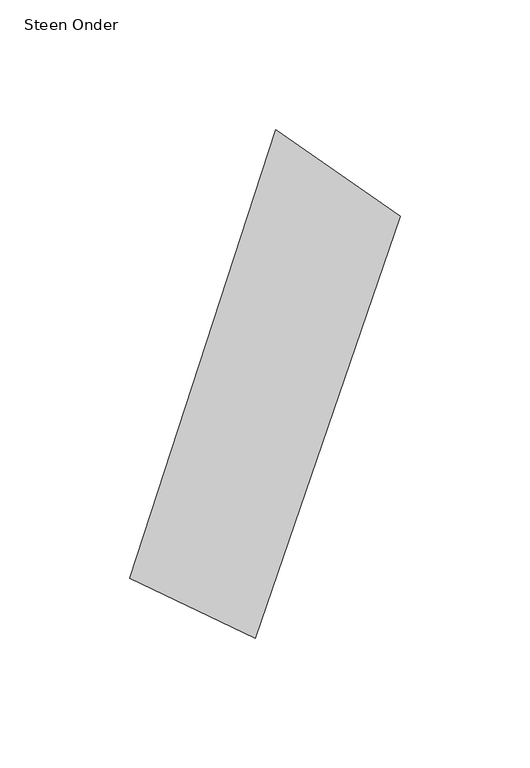
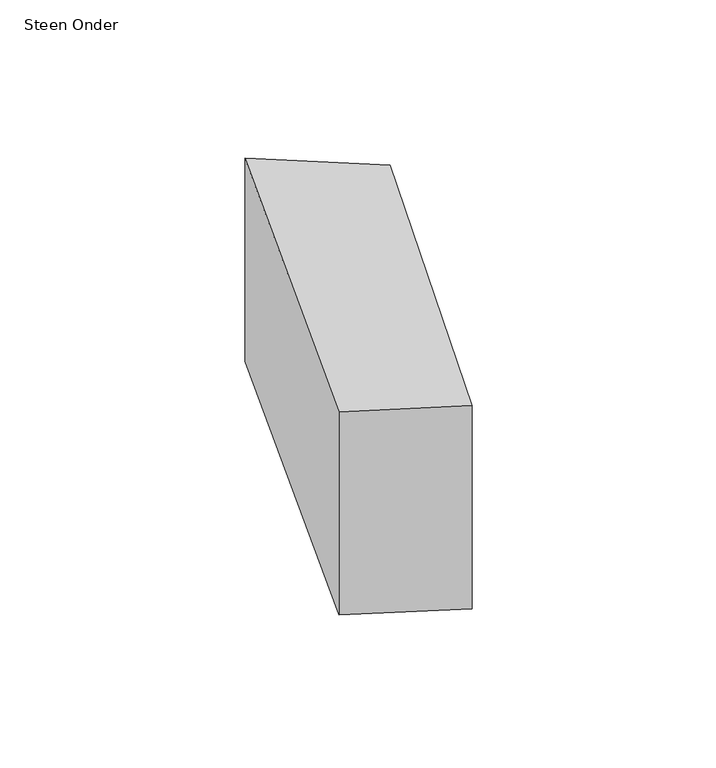
"""IFC4 building model written with IfcOpenShell, lengths in millimetres: proxy geometry, 00_GMA_steen_versie_4 : Steen Onder."""

from ifc_helpers import new_model, si_unit, origin, origin_with_axes, place, context, project, spatial, polyline, outline, extrude, source, transform, mapped, element, save


def steen_onder_437b1255(model_context):
    return source(origin(), model_context, "Body", "SweptSolid", [
        extrude(outline(polyline([(128.4601409, 150.3532833), (72.5592981, -12.5768616), (24.0540247, 10.5473174), (80.4171752, 183.7389284), (128.4601409, 150.3532833)])), origin_with_axes(), (0.0, 0.0, 1.0), 100.0),
    ])


if __name__ == "__main__":
    model = new_model("IFC4")
    model_context = context("Model", 3, world=origin())
    ifc_project = project(units=[si_unit("LENGTHUNIT", "METRE", prefix="MILLI")], contexts=[model_context])
    site = spatial("IfcSite", under=ifc_project)
    building = spatial("IfcBuilding", under=site)
    placement = place(None, origin())
    steen_onder_shape = steen_onder_437b1255(model_context)
    element("IfcBuildingElementProxy", 1, Name="00_GMA_steen_versie_4 : Steen Onder", ObjectType="00_GMA_steen_versie_4 : Steen Onder", at=placement, inside=building, context=model_context, shape_type="MappedRepresentation", body=[
        mapped(steen_onder_shape, transform((0.0, 0.0, 0.0), x_axis=(1.0, 0.0, 0.0), y_axis=(0.0, 1.0, 0.0), z_axis=(0.0, 0.0, 1.0))),
    ])
    save(model, "model.ifc")

# Revit data of these elements
# Type "00_GMA_steen_versie_4 : Steen Onder"
#   StootVoegHalfBoven [instance default] = 5 mm
#   StootVoegHalf [instance default] = 5 mm
#   StootVoegBreedteOnder = 10 mm
#   StootVoegBreedteBoven = 10 mm
#   Steendikte = 100 mm
#   LintVoegOnderHalf = 0 mm
#   LintVoegOnder = 0 mm
#   LintVoegBovenHalf = 5 mm
#   LintVoegBoven = 10 mm
#   materiaal = none
#   MateriaalVoeg = none
#   Default Elevation = 0
